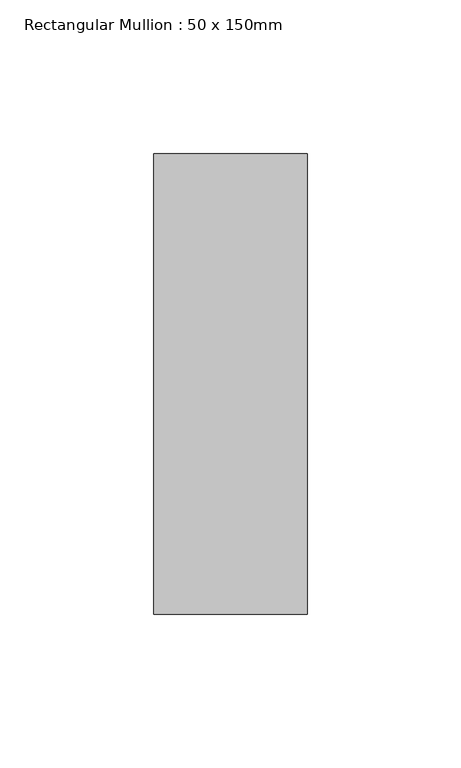
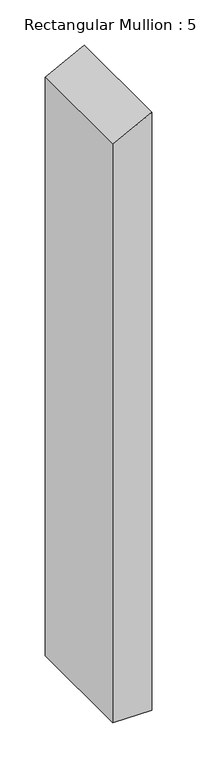
"""IFC4 building model written with IfcOpenShell, lengths in millimetres: member geometry, Rectangular Mullion : 50 x 150mm."""

from ifc_helpers import new_model, si_unit, frame, origin, place, context, project, spatial, polyline, outline, extrude, source, transform, mapped, element, save


def rectangular_mullion_50_x_150mm_c7e263e8(model_context):
    return source(origin(), model_context, "Body", "SweptSolid", [
        extrude(outline(polyline([(0.0, 0.0), (-26.0283525, -50.0), (-810.0622615, -50.0), (-810.0622615, 0.0), (0.0, 0.0)])), frame((0.0, -75.0, 0.0), z_axis=(0.0, 1.0, 0.0), x_axis=(0.0, 0.0, 1.0)), (0.0, 0.0, 1.0), 150.0),
    ])


if __name__ == "__main__":
    model = new_model("IFC4")
    model_context = context("Model", 3, world=origin())
    ifc_project = project(units=[si_unit("LENGTHUNIT", "METRE", prefix="MILLI")], contexts=[model_context])
    site = spatial("IfcSite", under=ifc_project)
    building = spatial("IfcBuilding", under=site)
    placement = place(None, origin())
    rectangular_mullion_50_x_150mm_shape = rectangular_mullion_50_x_150mm_c7e263e8(model_context)
    element("IfcMember", 1, ObjectType="Rectangular Mullion : 50 x 150mm", at=placement, inside=building, context=model_context, shape_type="MappedRepresentation", body=[
        mapped(rectangular_mullion_50_x_150mm_shape, transform((0.0, 0.0, 0.0), x_axis=(1.0, 0.0, 0.0), y_axis=(0.0, 1.0, 0.0), z_axis=(0.0, 0.0, 1.0))),
    ])
    save(model, "model.ifc")

# Revit data of these elements
# Type "Rectangular Mullion : 50 x 150mm"
#   built-in parameter 1007304 = 0.492126 (stored number, unit not read)
#   built-in parameter 1007301 = 0.082021 (stored number, unit not read)
#   built-in parameter 1007300 = 0.082021 (stored number, unit not read)
# Element 1 (IfcMember, "Rectangular Mullion : 50 x 150mm")
#   Materials on its faces: "Aluminium"
# Materials
#   "Aluminium": class "Metal", colour RGB 247 247 247, transparency 0, Description = "Aluminium 6061", Cost = 0
